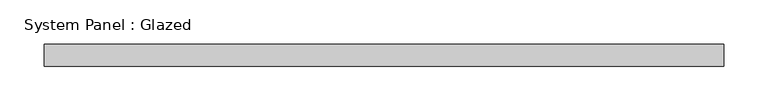
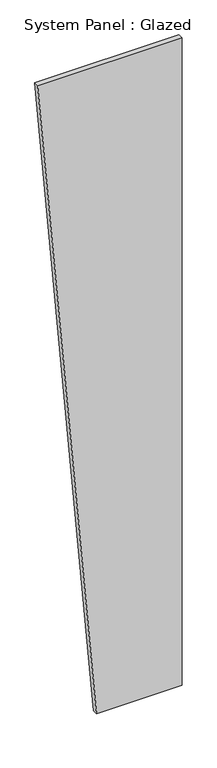
"""IFC4 building model written with IfcOpenShell, lengths in millimetres: plate geometry, System Panel : Glazed."""

from ifc_helpers import new_model, si_unit, frame, origin, place, context, project, spatial, polyline, outline, extrude, source, transform, mapped, element, save


def system_panel_glazed_35afb83b(model_context):
    return source(origin(), model_context, "Body", "SweptSolid", [
        extrude(outline(polyline([(0.0, -71.0314805), (0.0, 386.1685195), (3657.6, 386.1685195), (3657.6, -386.1685195), (0.0, -71.0314805)])), frame((0.0, -44.45, 0.0), z_axis=(0.0, 1.0, 0.0), x_axis=(0.0, 0.0, 1.0)), (0.0, 0.0, 1.0), 25.4),
    ])


if __name__ == "__main__":
    model = new_model("IFC4")
    model_context = context("Model", 3, world=origin())
    ifc_project = project(units=[si_unit("LENGTHUNIT", "METRE", prefix="MILLI")], contexts=[model_context])
    site = spatial("IfcSite", under=ifc_project)
    building = spatial("IfcBuilding", under=site)
    placement = place(None, origin())
    system_panel_glazed_shape = system_panel_glazed_35afb83b(model_context)
    element("IfcPlate", 1, ObjectType="System Panel : Glazed", at=placement, inside=building, context=model_context, shape_type="MappedRepresentation", body=[
        mapped(system_panel_glazed_shape, transform((0.0, 0.0, 0.0), x_axis=(1.0, 0.0, 0.0), y_axis=(0.0, 1.0, 0.0), z_axis=(0.0, 0.0, 1.0))),
    ])
    save(model, "model.ifc")

# Revit data of these elements
# Type "System Panel : Glazed"
#   Construction Type Id = "GSP4R"
#   Analytic Construction = "1/8 in Pilkington single glazing"
#   Visual Light Transmittance = 0.9
#   Solar Heat Gain Coefficient = 0.86
#   Heat Transfer Coefficient (U) = 1.18115 BTU/(h·ft²·°F)
#   Define Thermal Properties by = 1
# Element 1 (IfcPlate, "System Panel : Glazed")
#   Materials on its faces: "Glass"
# Materials
#   "Glass": class "Glass", colour RGB 0 128 192, transparency 0.75, Description = "Soda Lime Glass", Cost = 0
